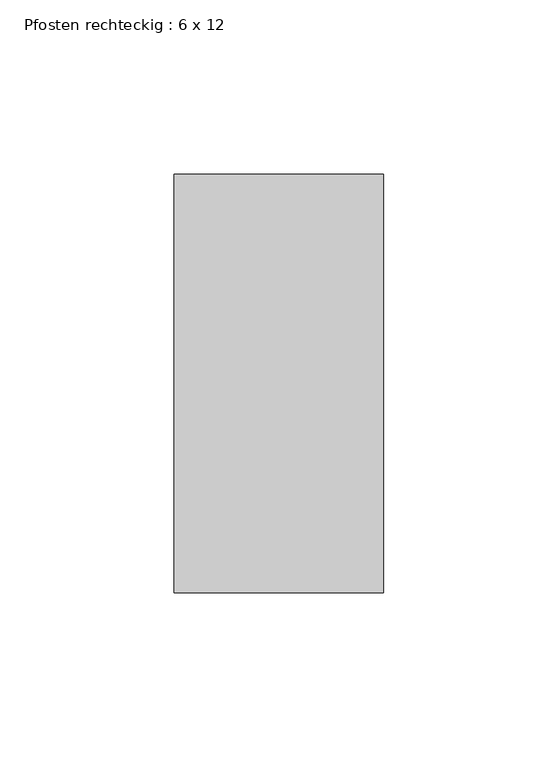
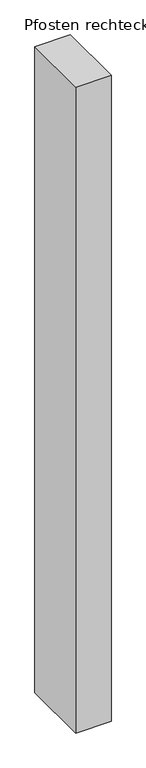
"""IFC4 building model written with IfcOpenShell, lengths in millimetres: member geometry, Pfosten rechteckig : 6 x 12."""

from ifc_helpers import new_model, si_unit, frame, origin, place, context, project, spatial, polyline, outline, extrude, source, transform, mapped, element, save


def pfosten_rechteckig_6_x_12_ce3c1f4b(model_context):
    return source(origin(), model_context, "Body", "SweptSolid", [
        extrude(outline(polyline([(30.0, 60.0), (30.0, -60.0), (-30.0, -60.0), (-30.0, 60.0), (30.0, 60.0)])), frame((0.0, 0.0, -1160.0000003), z_axis=(0.0, 0.0, 1.0), x_axis=(1.0, 0.0, 0.0)), (0.0, 0.0, 1.0), 1160.0000003),
    ])


if __name__ == "__main__":
    model = new_model("IFC4")
    model_context = context("Model", 3, world=origin())
    ifc_project = project(units=[si_unit("LENGTHUNIT", "METRE", prefix="MILLI")], contexts=[model_context])
    site = spatial("IfcSite", under=ifc_project)
    building = spatial("IfcBuilding", under=site)
    placement = place(None, origin())
    pfosten_rechteckig_6_x_12_shape = pfosten_rechteckig_6_x_12_ce3c1f4b(model_context)
    element("IfcMember", 1, ObjectType="Pfosten rechteckig : 6 x 12", at=placement, inside=building, context=model_context, shape_type="MappedRepresentation", body=[
        mapped(pfosten_rechteckig_6_x_12_shape, transform((0.0, 0.0, 0.0), x_axis=(1.0, 0.0, 0.0), y_axis=(0.0, 1.0, 0.0), z_axis=(0.0, 0.0, 1.0))),
    ])
    save(model, "model.ifc")

# Revit data of these elements
# Type "Pfosten rechteckig : 6 x 12"
#   built-in parameter 1007304 = 0.393701 (stored number, unit not read)
#   built-in parameter 1007301 = 0.0984252 (stored number, unit not read)
#   built-in parameter 1007300 = 0.0984252 (stored number, unit not read)
# Element 1 (IfcMember, "Pfosten rechteckig : 6 x 12")
#   Materials on its faces: "Metall - verzinkt"
# Materials
#   "Metall - verzinkt": class "Allgemeines", colour RGB 200 200 200, transparency 0, Cost = 0
